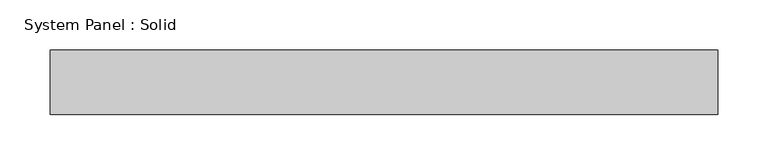
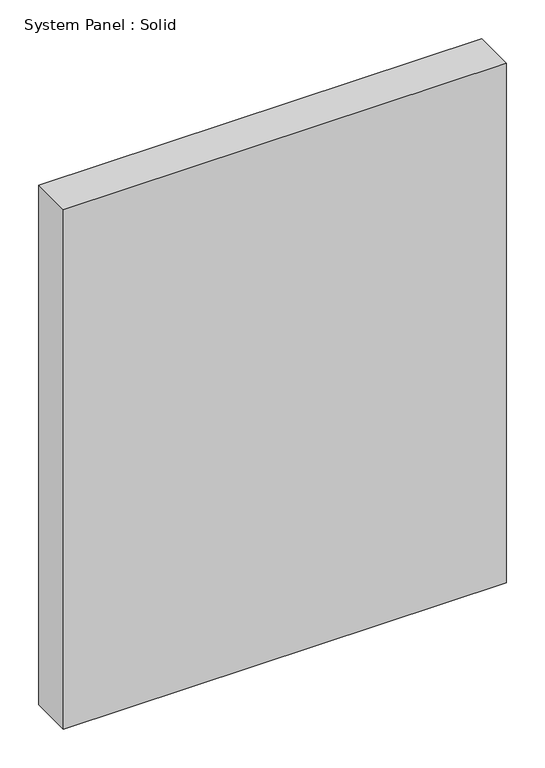
"""IFC4 building model written with IfcOpenShell, lengths in millimetres: plate geometry, System Panel : Solid."""

from ifc_helpers import new_model, si_unit, origin, origin_with_axes, place, context, project, spatial, polyline, outline, extrude, source, transform, mapped, element, save


def system_panel_solid_90d8cc78(model_context):
    return source(origin(), model_context, "Body", "SweptSolid", [
        extrude(outline(polyline([(330.2, -44.45), (-330.2, -44.45), (-330.2, 19.05), (330.2, 19.05), (330.2, -44.45)])), origin_with_axes(), (0.0, 0.0, 1.0), 819.15),
    ])


if __name__ == "__main__":
    model = new_model("IFC4")
    model_context = context("Model", 3, world=origin())
    ifc_project = project(units=[si_unit("LENGTHUNIT", "METRE", prefix="MILLI")], contexts=[model_context])
    site = spatial("IfcSite", under=ifc_project)
    building = spatial("IfcBuilding", under=site)
    placement = place(None, origin())
    system_panel_solid_shape = system_panel_solid_90d8cc78(model_context)
    element("IfcPlate", 1, ObjectType="System Panel : Solid", at=placement, inside=building, context=model_context, shape_type="MappedRepresentation", body=[
        mapped(system_panel_solid_shape, transform((0.0, 0.0, 0.0), x_axis=(1.0, 0.0, 0.0), y_axis=(0.0, 1.0, 0.0), z_axis=(0.0, 0.0, 1.0))),
    ])
    save(model, "model.ifc")

# Revit data of these elements
# Type "System Panel : Solid"
#   Construction Type Id = "MDOOR"
#   Analytic Construction = "Metal"
#   Visual Light Transmittance = 0
#   Solar Heat Gain Coefficient = 0
#   Heat Transfer Coefficient (U) = 0.651978 BTU/(h·ft²·°F)
#   Define Thermal Properties by = 1
# Element 1 (IfcPlate, "System Panel : Solid")
#   Materials on its faces: "Default"
# Materials
#   "Default": class "Miscellaneous", colour RGB 127 127 127, transparency 0, Cost = 0
